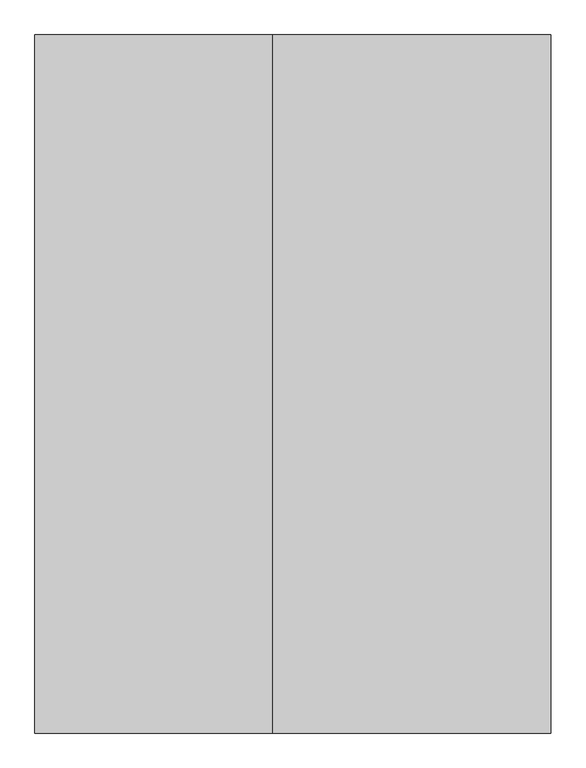
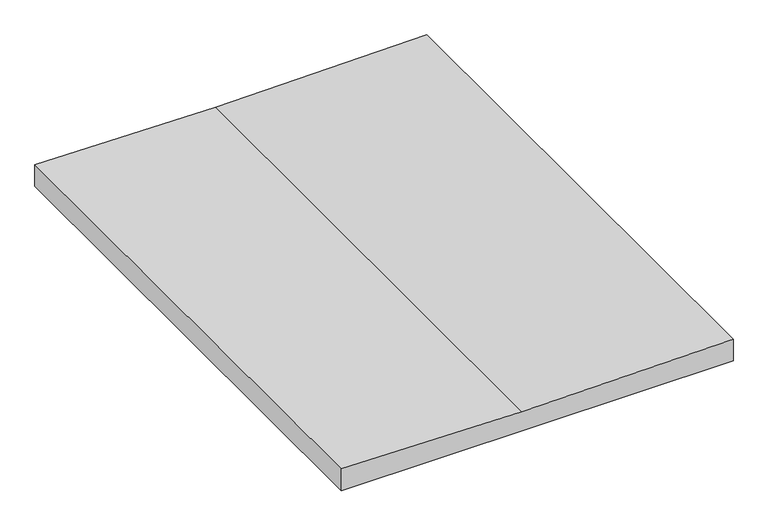
"""IFC4 building model written with IfcOpenShell, lengths in millimetres: proxy geometry, FIRESTONE INSULATION003 : FIRESTONE INSULATION003."""

from ifc_helpers import new_model, si_unit, frame, origin, place, context, project, spatial, polyline, outline, extrude, source, transform, mapped, element, save


def generic_models_44e1ce57(model_context):
    return source(origin(), model_context, "Body", "SweptSolid", [
        extrude(outline(polyline([(40131.746, -2567.3737014), (40131.746, -1090.0815411), (40218.4000089, -1090.0815411), (40208.6021556, -1886.5629484), (40218.4000089, -2567.3737014), (40131.746, -2567.3737014)])), frame((0.0, 1000.0, 0.0), z_axis=(0.0, 1.0, 0.0), x_axis=(0.0, 0.0, 1.0)), (0.0, 0.0, 1.0), 2000.0),
    ])


if __name__ == "__main__":
    model = new_model("IFC4")
    model_context = context("Model", 3, world=origin())
    ifc_project = project(units=[si_unit("LENGTHUNIT", "METRE", prefix="MILLI")], contexts=[model_context])
    site = spatial("IfcSite", under=ifc_project)
    building = spatial("IfcBuilding", under=site)
    placement = place(None, origin())
    generic_models_shape = generic_models_44e1ce57(model_context)
    element("IfcBuildingElementProxy", 1, Name="FIRESTONE INSULATION003 : FIRESTONE INSULATION003", ObjectType="FIRESTONE INSULATION003 : FIRESTONE INSULATION003", at=placement, inside=building, context=model_context, shape_type="MappedRepresentation", body=[
        mapped(generic_models_shape, transform((0.0, 0.0, 0.0), x_axis=(1.0, 0.0, 0.0), y_axis=(0.0, 1.0, 0.0), z_axis=(0.0, 0.0, 1.0))),
    ])
    save(model, "model.ifc")

# Revit data of these elements
# Type "FIRESTONE INSULATION003 : FIRESTONE INSULATION003"
#   NameOverride = "FIRESTONE INSULATION003"
# Element 1 (IfcBuildingElementProxy, "FIRESTONE INSULATION003 : FIRESTONE INSULATION003")
#   Materials on its faces: "TAPERED 2X SLEEPERS - SLOPED TO DRAIN"
# Materials
#   "TAPERED 2X SLEEPERS - SLOPED TO DRAIN": class "Unassigned", colour RGB 234 198 178, transparency 0
